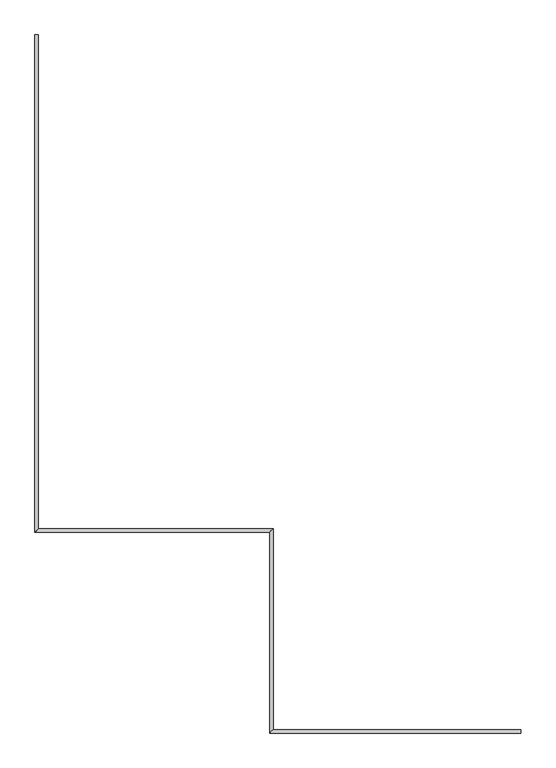
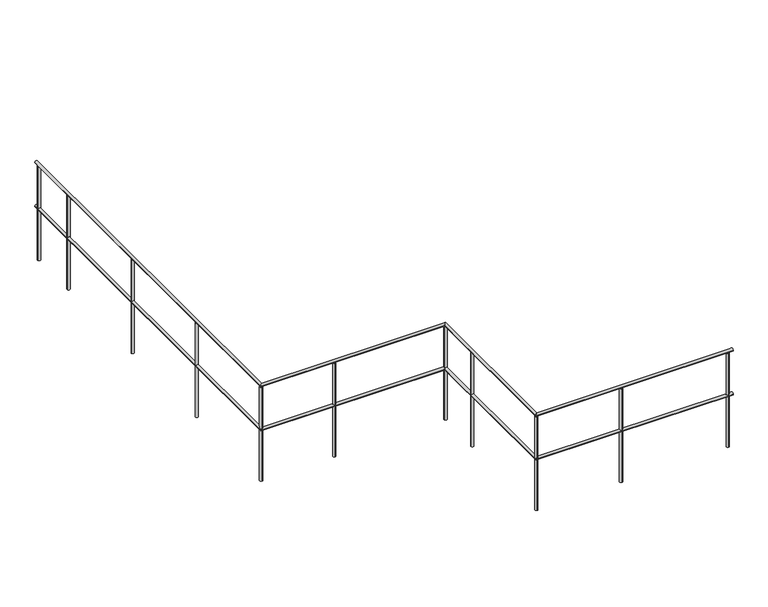
"""IFC4 building model written with IfcOpenShell, lengths in millimetres: railing geometry."""

import ifcopenshell
import ifcopenshell.guid

model = None  # the IFC model being written
_history = None  # IfcOwnerHistory: only IFC2X3 demands one
_inside = {}  # id of a spatial element -> (the spatial element, [elements in it])
_under = {}  # id of a project, library or spatial element -> (it, [spatial elements below it])
_declared = {}  # id of a project -> (the project, [libraries it declares])
_typed = {}  # id of a type object -> (the type object, [elements of that type])
_made_of = {}  # id of a material, layer set ... -> (it, [elements and type objects made of it])


def new_model(schema):
    """Start an empty IFC model of exactly this schema.

    Asked for "IFC4X3", IfcOpenShell would pick the latest addendum, in which some entities
    have other attributes; the version numbers below select the first issue.
    IFC2X3 requires an IfcOwnerHistory on every rooted entity: one is made here for all.
    """
    global model, _history
    if schema == "IFC4X3":
        model = ifcopenshell.file(schema_version=(4, 3, 0, 0))
    else:
        model = ifcopenshell.file(schema=schema)
    _inside.clear()
    _under.clear()
    _declared.clear()
    _typed.clear()
    _made_of.clear()
    _history = None
    if model.schema == "IFC2X3":
        org = make("IfcOrganization", Name="unknown")
        user = make(
            "IfcPersonAndOrganization",
            ThePerson=make("IfcPerson", FamilyName="unknown"),
            TheOrganization=org,
        )
        app = make(
            "IfcApplication",
            ApplicationDeveloper=org,
            Version="unknown",
            ApplicationFullName="unknown",
            ApplicationIdentifier="unknown",
        )
        _history = make(
            "IfcOwnerHistory",
            OwningUser=user,
            OwningApplication=app,
            ChangeAction="ADDED",
            CreationDate=0,
        )
    return model


def make(cls, **values):
    """One entity of the class cls with the attributes given. An attribute that is None is left unset."""
    return model.create_entity(
        cls, **{name: value for name, value in values.items() if value is not None}
    )


def rooted(cls, **values):
    """An entity with a GlobalId (a new one), such as an element, a storey or a relation."""
    return make(cls, GlobalId=ifcopenshell.guid.new(), OwnerHistory=_history, **values)


def si_unit(unit_type, name, prefix=None):
    """IfcSIUnit, for example si_unit("LENGTHUNIT", "METRE", prefix="MILLI")."""
    return make("IfcSIUnit", UnitType=unit_type, Prefix=prefix, Name=name)


def assignment(units):
    """IfcUnitAssignment: the units of a project."""
    return None if units is None else make("IfcUnitAssignment", Units=units)


def point(xyz):
    """IfcCartesianPoint."""
    return None if xyz is None else make("IfcCartesianPoint", Coordinates=xyz)


def direction(xyz):
    """IfcDirection."""
    return None if xyz is None else make("IfcDirection", DirectionRatios=xyz)


def frame(location, z_axis=None, x_axis=None):
    """IfcAxis2Placement3D, a coordinate frame: its origin and axes. An axis left out is left unset."""
    return make(
        "IfcAxis2Placement3D",
        Location=point(location),
        Axis=direction(z_axis),
        RefDirection=direction(x_axis),
    )


def frame_2d(location, x_axis=None):
    """IfcAxis2Placement2D, a coordinate frame in the plane: its origin and x axis."""
    return make(
        "IfcAxis2Placement2D", Location=point(location), RefDirection=direction(x_axis)
    )


def origin():
    """The frame at (0, 0, 0) with its axes left unset."""
    return frame((0.0, 0.0, 0.0))


def place(relative_to, where):
    """IfcLocalPlacement: puts the frame where relative to a parent placement (None: the world)."""
    return make(
        "IfcLocalPlacement", PlacementRelTo=relative_to, RelativePlacement=where
    )


def context(
    kind, dimensions, precision=None, world=None, true_north=None, identifier=None
):
    """IfcGeometricRepresentationContext, for example the 3D "Model" context."""
    return make(
        "IfcGeometricRepresentationContext",
        ContextIdentifier=identifier,
        ContextType=kind,
        CoordinateSpaceDimension=dimensions,
        Precision=precision,
        WorldCoordinateSystem=world,
        TrueNorth=true_north,
    )


def project(units=None, contexts=None):
    """IfcProject with its units and contexts."""
    return rooted(
        "IfcProject",
        Name="project",
        RepresentationContexts=contexts,
        UnitsInContext=assignment(units),
    )


def spatial(cls, under=None, at=None, **own):
    """A site, building, storey or space (cls), placed at a placement, below another one or the project."""
    s = rooted(cls, ObjectPlacement=at, **own)
    if under is not None:
        _under.setdefault(under.id(), (under, []))[1].append(s)
    return s


def circle_curve(where, radius):
    """IfcCircle in the frame where."""
    return make("IfcCircle", Position=where, Radius=radius)


def ellipse_curve(where, semi_axis1, semi_axis2):
    """IfcEllipse in the frame where."""
    return make(
        "IfcEllipse", Position=where, SemiAxis1=semi_axis1, SemiAxis2=semi_axis2
    )


def trimmed(basis, trim1, trim2, sense, master):
    """IfcTrimmedCurve: the piece of a basis curve between two trims."""
    return make(
        "IfcTrimmedCurve",
        BasisCurve=basis,
        Trim1=trim1,
        Trim2=trim2,
        SenseAgreement=sense,
        MasterRepresentation=master,
    )


def segment(curve, same_sense, transition):
    """IfcCompositeCurveSegment."""
    return make(
        "IfcCompositeCurveSegment",
        Transition=transition,
        SameSense=same_sense,
        ParentCurve=curve,
    )


def composite_curve(segments, self_intersect=None):
    """IfcCompositeCurve: segments joined end to end."""
    return make("IfcCompositeCurve", Segments=segments, SelfIntersect=self_intersect)


def outline(outer, holes=None, kind="AREA"):
    """IfcArbitraryClosedProfileDef: a profile drawn as a closed curve; with holes, ...WithVoids."""
    if holes is None:
        return make("IfcArbitraryClosedProfileDef", ProfileType=kind, OuterCurve=outer)
    return make(
        "IfcArbitraryProfileDefWithVoids",
        ProfileType=kind,
        OuterCurve=outer,
        InnerCurves=holes,
    )


def extrude(swept, where, along, depth):
    """IfcExtrudedAreaSolid: the profile swept, set in the frame where, extruded along a direction by depth."""
    return make(
        "IfcExtrudedAreaSolid",
        SweptArea=swept,
        Position=where,
        ExtrudedDirection=direction(along),
        Depth=depth,
    )


def shape(context_of_items, identifier, shape_type, items):
    """IfcShapeRepresentation: the items that make up one representation, for example the "Body"."""
    return make(
        "IfcShapeRepresentation",
        ContextOfItems=context_of_items,
        RepresentationIdentifier=identifier,
        RepresentationType=shape_type,
        Items=items,
    )


def source(mapping_origin, context_of_items, identifier, shape_type, items):
    """IfcRepresentationMap: a shape defined once, which mapped items show again and again."""
    return make(
        "IfcRepresentationMap",
        MappingOrigin=mapping_origin,
        MappedRepresentation=shape(context_of_items, identifier, shape_type, items),
    )


def transform(
    local_origin,
    x_axis=None,
    y_axis=None,
    z_axis=None,
    scale=None,
    scale2=None,
    scale3=None,
    uniform=True,
):
    """IfcCartesianTransformationOperator3D, or its non-uniform kind. x_axis, y_axis, z_axis: its Axis1, 2, 3."""
    if uniform:
        return make(
            "IfcCartesianTransformationOperator3D",
            Axis1=direction(x_axis),
            Axis2=direction(y_axis),
            LocalOrigin=point(local_origin),
            Scale=scale,
            Axis3=direction(z_axis),
        )
    return make(
        "IfcCartesianTransformationOperator3DnonUniform",
        Axis1=direction(x_axis),
        Axis2=direction(y_axis),
        LocalOrigin=point(local_origin),
        Scale=scale,
        Axis3=direction(z_axis),
        Scale2=scale2,
        Scale3=scale3,
    )


def mapped(mapping_source, mapping_target):
    """IfcMappedItem: shows the shape of a source again, moved by a transform."""
    return make(
        "IfcMappedItem", MappingSource=mapping_source, MappingTarget=mapping_target
    )


def made_of(thing, what):
    """Note that an element or type object is made of a material, layer set ...; save() writes the relation."""
    if what is not None:
        _made_of.setdefault(what.id(), (what, []))[1].append(thing)
    return thing


def element(
    cls,
    number,
    at=None,
    inside=None,
    cuts=None,
    type_object=None,
    material=None,
    context=None,
    identifier="Body",
    shape_type=None,
    held_by="IfcProductDefinitionShape",
    body=None,
    shapes=None,
    **own,
):
    """One element of the class cls, such as IfcWall. Its Tag is "e" and its number.

    at: its placement. inside: the storey or other place that contains it. cuts: it is an
    opening in that element (IfcRelVoidsElement). A single representation is given by context,
    identifier, shape_type and body (its items); several are given by shapes. held_by: the class
    of the entity that holds the representations. save() writes the other relations.
    """
    e = rooted(cls, Tag="e%d" % number, ObjectPlacement=at, **own)
    if body is not None:
        shapes = [shape(context, identifier, shape_type, body)]
    if shapes is not None:
        e.Representation = make(held_by, Representations=shapes)
    if inside is not None:
        _inside.setdefault(inside.id(), (inside, []))[1].append(e)
    if cuts is not None:
        rooted(
            "IfcRelVoidsElement", RelatingBuildingElement=cuts, RelatedOpeningElement=e
        )
    if type_object is not None:
        _typed.setdefault(type_object.id(), (type_object, []))[1].append(e)
    return made_of(e, material)


def aggregate(whole, parts):
    """IfcRelAggregates: a whole, such as a stair, and the parts it consists of."""
    return rooted("IfcRelAggregates", RelatingObject=whole, RelatedObjects=parts)


def save(model, path):
    """Write the relations noted so far, then the file.

    IfcRelAggregates (storeys below a building ...), IfcRelContainedInSpatialStructure (elements
    in a storey), IfcRelDefinesByType, IfcRelAssociatesMaterial and IfcRelDeclares: one each for
    every whole, place, type object, material and project.
    """
    for whole, parts in _under.values():
        aggregate(whole, parts)
    for where, things in _inside.values():
        rooted(
            "IfcRelContainedInSpatialStructure",
            RelatedElements=things,
            RelatingStructure=where,
        )
    for kind, things in _typed.values():
        rooted("IfcRelDefinesByType", RelatedObjects=things, RelatingType=kind)
    for what, things in _made_of.values():
        rooted("IfcRelAssociatesMaterial", RelatedObjects=things, RelatingMaterial=what)
    for by, libraries in _declared.values():
        rooted("IfcRelDeclares", RelatingContext=by, RelatedDefinitions=libraries)
    model.write(path)


def plane_surface(at):
    """IfcPlane: the flat surface through the origin of the frame at, square to its z axis."""
    return make("IfcPlane", Position=at)


def cylinder_surface(at, radius):
    """IfcCylindricalSurface: all points at the distance radius from the z axis of the frame at."""
    return make("IfcCylindricalSurface", Position=at, Radius=radius)


def advanced_brep(points, edges, surfaces, faces):
    """IfcAdvancedBrep: a solid bounded by faces that lie on surfaces and meet in shared edges.

    An edge is (start, end): straight between two places in points (the first is 0);
    or (start, end, curve); or (start, end, curve, False) where it runs against its curve.
    A face is (place in surfaces, loops), or (place, loops, False) where it looks against
    its surface's normal. A loop lists edges by number (the first is 1), with a minus sign
    where the edge is run from its end to its start. The first loop is the outer one.
    """
    corners = [point(p) for p in points]
    vertices = [make("IfcVertexPoint", VertexGeometry=c) for c in corners]
    made = []
    for start, end, *more in edges:
        made.append(
            make(
                "IfcEdgeCurve",
                EdgeStart=vertices[start],
                EdgeEnd=vertices[end],
                EdgeGeometry=more[0] if more else make("IfcPolyline", Points=[corners[start], corners[end]]),
                SameSense=more[1] if len(more) > 1 else True,
            )
        )
    hull = []
    for where, loops, *sense in faces:
        bounds = []
        for j, loop in enumerate(loops):
            ring = [make("IfcOrientedEdge", EdgeElement=made[abs(k) - 1], Orientation=k > 0) for k in loop]
            bounds.append(
                make(
                    "IfcFaceOuterBound" if j == 0 else "IfcFaceBound",
                    Bound=make("IfcEdgeLoop", EdgeList=ring),
                    Orientation=True,
                )
            )
        hull.append(make("IfcAdvancedFace", Bounds=bounds, FaceSurface=surfaces[where], SameSense=sense[0] if sense else True))
    return make("IfcAdvancedBrep", Outer=make("IfcClosedShell", CfsFaces=hull))


def railing_3c83800e(model_context):
    return source(origin(), model_context, "Body", "SolidModel", [
        advanced_brep(
        [(26040.0, -5867.9791411, 885.0), (26040.0, -5837.9791411, 885.0), (23912.0, -5867.9791411, 885.0), (23942.0, -5837.9791411, 885.0), (23912.0, -4167.9791411, 885.0), (23942.0, -4137.9791411, 885.0), (21924.0, -4167.9791411, 885.0), (21954.0, -4137.9791411, 885.0), (21924.0, 47.0208589, 885.0), (21954.0, 47.0208589, 885.0)],
        [
            (0, 1, circle_curve(frame((26040.0, -5852.9791411, 885.0), z_axis=(1.0, 0.0, 0.0), x_axis=(0.0, 1.0, 0.0)), 15.0)),
            (1, 0, circle_curve(frame((26040.0, -5852.9791411, 885.0), z_axis=(1.0, 0.0, 0.0), x_axis=(0.0, 1.0, 0.0)), 15.0)),
            (0, 2),
            (2, 3, ellipse_curve(frame((23927.0, -5852.9791411, 885.0), z_axis=(0.7071067811865454, -0.7071067811865496, 0.0), x_axis=(0.7071067811865498, 0.7071067811865452, 0.0)), 21.2132034, 15.0)),
            (3, 1),
            (3, 2, ellipse_curve(frame((23927.0, -5852.9791411, 885.0), z_axis=(0.7071067811865454, -0.7071067811865496, 0.0), x_axis=(0.7071067811865498, 0.7071067811865452, 0.0)), 21.2132034, 15.0)),
            (2, 4),
            (4, 5, ellipse_curve(frame((23927.0, -4152.9791411, 885.0), z_axis=(0.7071067811865454, -0.7071067811865497, 0.0), x_axis=(-0.7071067811865497, -0.7071067811865454, 0.0)), 21.2132034, 15.0)),
            (5, 3),
            (5, 4, ellipse_curve(frame((23927.0, -4152.9791411, 885.0), z_axis=(0.7071067811865454, -0.7071067811865497, 0.0), x_axis=(-0.7071067811865497, -0.7071067811865454, 0.0)), 21.2132034, 15.0)),
            (4, 6),
            (6, 7, ellipse_curve(frame((21939.0, -4152.9791411, 885.0), z_axis=(0.7071067811865455, -0.7071067811865496, 0.0), x_axis=(0.7071067811865495, 0.7071067811865455, 0.0)), 21.2132034, 15.0)),
            (7, 5),
            (7, 6, ellipse_curve(frame((21939.0, -4152.9791411, 885.0), z_axis=(0.7071067811865455, -0.7071067811865496, 0.0), x_axis=(0.7071067811865495, 0.7071067811865455, 0.0)), 21.2132034, 15.0)),
            (8, 9, circle_curve(frame((21939.0, 47.0208589, 885.0), z_axis=(0.0, 1.0, 0.0), x_axis=(1.0, 0.0, 0.0)), 15.0)),
            (9, 8, circle_curve(frame((21939.0, 47.0208589, 885.0), z_axis=(0.0, 1.0, 0.0), x_axis=(1.0, 0.0, 0.0)), 15.0)),
            (6, 8),
            (9, 7),
        ],
        [
            plane_surface(frame((26040.0, -5852.9791411, 900.0), z_axis=(1.0, 0.0, 0.0), x_axis=(0.0, -1.0, 0.0))),
            cylinder_surface(frame((26040.0, -5852.9791411, 885.0), z_axis=(1.0, 0.0, 0.0), x_axis=(0.0, 1.0, 0.0)), 15.0),
            cylinder_surface(frame((23927.0, -5852.9791411, 885.0), z_axis=(0.0, -1.0, 0.0), x_axis=(1.0, 0.0, 0.0)), 15.0),
            cylinder_surface(frame((23927.0, -4152.9791411, 885.0), z_axis=(1.0, 0.0, 0.0), x_axis=(0.0, 1.0, 0.0)), 15.0),
            plane_surface(frame((21939.0, 47.0208589, 900.0), z_axis=(0.0, 1.0, 0.0), x_axis=(0.0, 0.0, 1.0))),
            cylinder_surface(frame((21939.0, -4152.9791411, 885.0), z_axis=(0.0, -1.0, 0.0), x_axis=(1.0, 0.0, 0.0)), 15.0),
        ],
        [
            (0, [[1, 2]]),
            (1, [[-1, 3, 4, 5]]),
            (1, [[-2, -5, 6, -3]]),
            (2, [[-4, 7, 8, 9]]),
            (2, [[-6, -9, 10, -7]]),
            (3, [[-8, 11, 12, 13]]),
            (3, [[-10, -13, 14, -11]]),
            (4, [[15, 16]]),
            (5, [[-12, 17, -16, 18]]),
            (5, [[-14, -18, -15, -17]]),
        ],
    ),
        advanced_brep(
        [(26040.0, -5867.9791411, 1385.0), (26040.0, -5837.9791411, 1385.0), (23912.0, -5867.9791411, 1385.0), (23942.0, -5837.9791411, 1385.0), (23912.0, -4167.9791411, 1385.0), (23942.0, -4137.9791411, 1385.0), (21924.0, -4167.9791411, 1385.0), (21954.0, -4137.9791411, 1385.0), (21924.0, 47.0208589, 1385.0), (21954.0, 47.0208589, 1385.0)],
        [
            (0, 1, circle_curve(frame((26040.0, -5852.9791411, 1385.0), z_axis=(1.0, 0.0, 0.0), x_axis=(0.0, 1.0, 0.0)), 15.0)),
            (1, 0, circle_curve(frame((26040.0, -5852.9791411, 1385.0), z_axis=(1.0, 0.0, 0.0), x_axis=(0.0, 1.0, 0.0)), 15.0)),
            (0, 2),
            (2, 3, ellipse_curve(frame((23927.0, -5852.9791411, 1385.0), z_axis=(0.7071067811865454, -0.7071067811865496, 0.0), x_axis=(0.7071067811865498, 0.7071067811865452, 0.0)), 21.2132034, 15.0)),
            (3, 1),
            (3, 2, ellipse_curve(frame((23927.0, -5852.9791411, 1385.0), z_axis=(0.7071067811865454, -0.7071067811865496, 0.0), x_axis=(0.7071067811865498, 0.7071067811865452, 0.0)), 21.2132034, 15.0)),
            (2, 4),
            (4, 5, ellipse_curve(frame((23927.0, -4152.9791411, 1385.0), z_axis=(0.7071067811865454, -0.7071067811865497, 0.0), x_axis=(-0.7071067811865497, -0.7071067811865454, 0.0)), 21.2132034, 15.0)),
            (5, 3),
            (5, 4, ellipse_curve(frame((23927.0, -4152.9791411, 1385.0), z_axis=(0.7071067811865454, -0.7071067811865497, 0.0), x_axis=(-0.7071067811865497, -0.7071067811865454, 0.0)), 21.2132034, 15.0)),
            (4, 6),
            (6, 7, ellipse_curve(frame((21939.0, -4152.9791411, 1385.0), z_axis=(0.7071067811865455, -0.7071067811865496, 0.0), x_axis=(0.7071067811865495, 0.7071067811865455, 0.0)), 21.2132034, 15.0)),
            (7, 5),
            (7, 6, ellipse_curve(frame((21939.0, -4152.9791411, 1385.0), z_axis=(0.7071067811865455, -0.7071067811865496, 0.0), x_axis=(0.7071067811865495, 0.7071067811865455, 0.0)), 21.2132034, 15.0)),
            (8, 9, circle_curve(frame((21939.0, 47.0208589, 1385.0), z_axis=(0.0, 1.0, 0.0), x_axis=(1.0, 0.0, 0.0)), 15.0)),
            (9, 8, circle_curve(frame((21939.0, 47.0208589, 1385.0), z_axis=(0.0, 1.0, 0.0), x_axis=(1.0, 0.0, 0.0)), 15.0)),
            (6, 8),
            (9, 7),
        ],
        [
            plane_surface(frame((26040.0, -5852.9791411, 1400.0), z_axis=(1.0, 0.0, 0.0), x_axis=(0.0, -1.0, 0.0))),
            cylinder_surface(frame((26040.0, -5852.9791411, 1385.0), z_axis=(1.0, 0.0, 0.0), x_axis=(0.0, 1.0, 0.0)), 15.0),
            cylinder_surface(frame((23927.0, -5852.9791411, 1385.0), z_axis=(0.0, -1.0, 0.0), x_axis=(1.0, 0.0, 0.0)), 15.0),
            cylinder_surface(frame((23927.0, -4152.9791411, 1385.0), z_axis=(1.0, 0.0, 0.0), x_axis=(0.0, 1.0, 0.0)), 15.0),
            plane_surface(frame((21939.0, 47.0208589, 1400.0), z_axis=(0.0, 1.0, 0.0), x_axis=(0.0, 0.0, 1.0))),
            cylinder_surface(frame((21939.0, -4152.9791411, 1385.0), z_axis=(0.0, -1.0, 0.0), x_axis=(1.0, 0.0, 0.0)), 15.0),
        ],
        [
            (0, [[1, 2]]),
            (1, [[-1, 3, 4, 5]]),
            (1, [[-2, -5, 6, -3]]),
            (2, [[-4, 7, 8, 9]]),
            (2, [[-6, -9, 10, -7]]),
            (3, [[-8, 11, 12, 13]]),
            (3, [[-10, -13, 14, -11]]),
            (4, [[15, 16]]),
            (5, [[-12, 17, -16, 18]]),
            (5, [[-14, -18, -15, -17]]),
        ],
    ),
        extrude(outline(composite_curve([segment(trimmed(circle_curve(frame_2d((21939.0, -552.9791411)), 15.0), [point((21924.0, -552.9791411))], [point((21954.0, -552.9791411))], False, "CARTESIAN"), True, "CONTINUOUS"), segment(trimmed(circle_curve(frame_2d((21939.0, -552.9791411)), 15.0), [point((21954.0, -552.9791411))], [point((21924.0, -552.9791411))], False, "CARTESIAN"), True, "CONTINUOUS")], self_intersect=False)), frame((0.0, 0.0, 300.0), z_axis=(0.0, 0.0, 1.0), x_axis=(1.0, 0.0, 0.0)), (0.0, 0.0, 1.0), 1070.0),
        extrude(outline(composite_curve([segment(trimmed(circle_curve(frame_2d((21939.0, -1752.9791411)), 15.0), [point((21924.0, -1752.9791411))], [point((21954.0, -1752.9791411))], False, "CARTESIAN"), True, "CONTINUOUS"), segment(trimmed(circle_curve(frame_2d((21939.0, -1752.9791411)), 15.0), [point((21954.0, -1752.9791411))], [point((21924.0, -1752.9791411))], False, "CARTESIAN"), True, "CONTINUOUS")], self_intersect=False)), frame((0.0, 0.0, 300.0), z_axis=(0.0, 0.0, 1.0), x_axis=(1.0, 0.0, 0.0)), (0.0, 0.0, 1.0), 1070.0),
        extrude(outline(composite_curve([segment(trimmed(circle_curve(frame_2d((21939.0, -2952.9791411)), 15.0), [point((21924.0, -2952.9791411))], [point((21954.0, -2952.9791411))], False, "CARTESIAN"), True, "CONTINUOUS"), segment(trimmed(circle_curve(frame_2d((21939.0, -2952.9791411)), 15.0), [point((21954.0, -2952.9791411))], [point((21924.0, -2952.9791411))], False, "CARTESIAN"), True, "CONTINUOUS")], self_intersect=False)), frame((0.0, 0.0, 300.0), z_axis=(0.0, 0.0, 1.0), x_axis=(1.0, 0.0, 0.0)), (0.0, 0.0, 1.0), 1070.0),
        extrude(outline(composite_curve([segment(trimmed(circle_curve(frame_2d((22727.0, -4152.9791411)), 15.0), [point((22727.0, -4167.9791411))], [point((22727.0, -4137.9791411))], False, "CARTESIAN"), True, "CONTINUOUS"), segment(trimmed(circle_curve(frame_2d((22727.0, -4152.9791411)), 15.0), [point((22727.0, -4137.9791411))], [point((22727.0, -4167.9791411))], False, "CARTESIAN"), True, "CONTINUOUS")], self_intersect=False)), frame((0.0, 0.0, 300.0), z_axis=(0.0, 0.0, 1.0), x_axis=(1.0, 0.0, 0.0)), (0.0, 0.0, 1.0), 1070.0),
        extrude(outline(composite_curve([segment(trimmed(circle_curve(frame_2d((23927.0, -4652.9791411)), 15.0), [point((23912.0, -4652.9791411))], [point((23942.0, -4652.9791411))], False, "CARTESIAN"), True, "CONTINUOUS"), segment(trimmed(circle_curve(frame_2d((23927.0, -4652.9791411)), 15.0), [point((23942.0, -4652.9791411))], [point((23912.0, -4652.9791411))], False, "CARTESIAN"), True, "CONTINUOUS")], self_intersect=False)), frame((0.0, 0.0, 300.0), z_axis=(0.0, 0.0, 1.0), x_axis=(1.0, 0.0, 0.0)), (0.0, 0.0, 1.0), 1070.0),
        extrude(outline(composite_curve([segment(trimmed(circle_curve(frame_2d((24840.0, -5852.9791411)), 15.0), [point((24840.0, -5867.9791411))], [point((24840.0, -5837.9791411))], False, "CARTESIAN"), True, "CONTINUOUS"), segment(trimmed(circle_curve(frame_2d((24840.0, -5852.9791411)), 15.0), [point((24840.0, -5837.9791411))], [point((24840.0, -5867.9791411))], False, "CARTESIAN"), True, "CONTINUOUS")], self_intersect=False)), frame((0.0, 0.0, 300.0), z_axis=(0.0, 0.0, 1.0), x_axis=(1.0, 0.0, 0.0)), (0.0, 0.0, 1.0), 1070.0),
        extrude(outline(composite_curve([segment(trimmed(circle_curve(frame_2d((21939.0, -4152.9791411)), 15.0), [point((21939.0, -4167.9791411))], [point((21939.0, -4137.9791411))], False, "CARTESIAN"), True, "CONTINUOUS"), segment(trimmed(circle_curve(frame_2d((21939.0, -4152.9791411)), 15.0), [point((21939.0, -4137.9791411))], [point((21939.0, -4167.9791411))], False, "CARTESIAN"), True, "CONTINUOUS")], self_intersect=False)), frame((0.0, 0.0, 300.0), z_axis=(0.0, 0.0, 1.0), x_axis=(1.0, 0.0, 0.0)), (0.0, 0.0, 1.0), 1070.0),
        extrude(outline(composite_curve([segment(trimmed(circle_curve(frame_2d((23927.0, -4152.9791411)), 15.0), [point((23912.0, -4152.9791411))], [point((23942.0, -4152.9791411))], False, "CARTESIAN"), True, "CONTINUOUS"), segment(trimmed(circle_curve(frame_2d((23927.0, -4152.9791411)), 15.0), [point((23942.0, -4152.9791411))], [point((23912.0, -4152.9791411))], False, "CARTESIAN"), True, "CONTINUOUS")], self_intersect=False)), frame((0.0, 0.0, 300.0), z_axis=(0.0, 0.0, 1.0), x_axis=(1.0, 0.0, 0.0)), (0.0, 0.0, 1.0), 1070.0),
        extrude(outline(composite_curve([segment(trimmed(circle_curve(frame_2d((23927.0, -5852.9791411)), 15.0), [point((23927.0, -5867.9791411))], [point((23927.0, -5837.9791411))], False, "CARTESIAN"), True, "CONTINUOUS"), segment(trimmed(circle_curve(frame_2d((23927.0, -5852.9791411)), 15.0), [point((23927.0, -5837.9791411))], [point((23927.0, -5867.9791411))], False, "CARTESIAN"), True, "CONTINUOUS")], self_intersect=False)), frame((0.0, 0.0, 300.0), z_axis=(0.0, 0.0, 1.0), x_axis=(1.0, 0.0, 0.0)), (0.0, 0.0, 1.0), 1070.0),
        extrude(outline(composite_curve([segment(trimmed(circle_curve(frame_2d((21939.0, -2.9791411)), 15.0), [point((21924.0, -2.9791411))], [point((21954.0, -2.9791411))], False, "CARTESIAN"), True, "CONTINUOUS"), segment(trimmed(circle_curve(frame_2d((21939.0, -2.9791411)), 15.0), [point((21954.0, -2.9791411))], [point((21924.0, -2.9791411))], False, "CARTESIAN"), True, "CONTINUOUS")], self_intersect=False)), frame((0.0, 0.0, 300.0), z_axis=(0.0, 0.0, 1.0), x_axis=(1.0, 0.0, 0.0)), (0.0, 0.0, 1.0), 1070.0),
        extrude(outline(composite_curve([segment(trimmed(circle_curve(frame_2d((25990.0, -5852.9791411)), 15.0), [point((25990.0, -5867.9791411))], [point((25990.0, -5837.9791411))], False, "CARTESIAN"), True, "CONTINUOUS"), segment(trimmed(circle_curve(frame_2d((25990.0, -5852.9791411)), 15.0), [point((25990.0, -5837.9791411))], [point((25990.0, -5867.9791411))], False, "CARTESIAN"), True, "CONTINUOUS")], self_intersect=False)), frame((0.0, 0.0, 300.0), z_axis=(0.0, 0.0, 1.0), x_axis=(1.0, 0.0, 0.0)), (0.0, 0.0, 1.0), 1070.0),
    ])


if __name__ == "__main__":
    model = new_model("IFC4")
    model_context = context("Model", 3, world=origin())
    ifc_project = project(units=[si_unit("LENGTHUNIT", "METRE", prefix="MILLI")], contexts=[model_context])
    site = spatial("IfcSite", under=ifc_project)
    building = spatial("IfcBuilding", under=site)
    placement = place(None, origin())
    railing_shape = railing_3c83800e(model_context)
    element("IfcRailing", 1, at=placement, inside=building, context=model_context, shape_type="MappedRepresentation", body=[
        mapped(railing_shape, transform((0.0, 0.0, 0.0), x_axis=(1.0, 0.0, 0.0), y_axis=(0.0, 1.0, 0.0), z_axis=(0.0, 0.0, 1.0))),
    ])
    save(model, "model.ifc")
